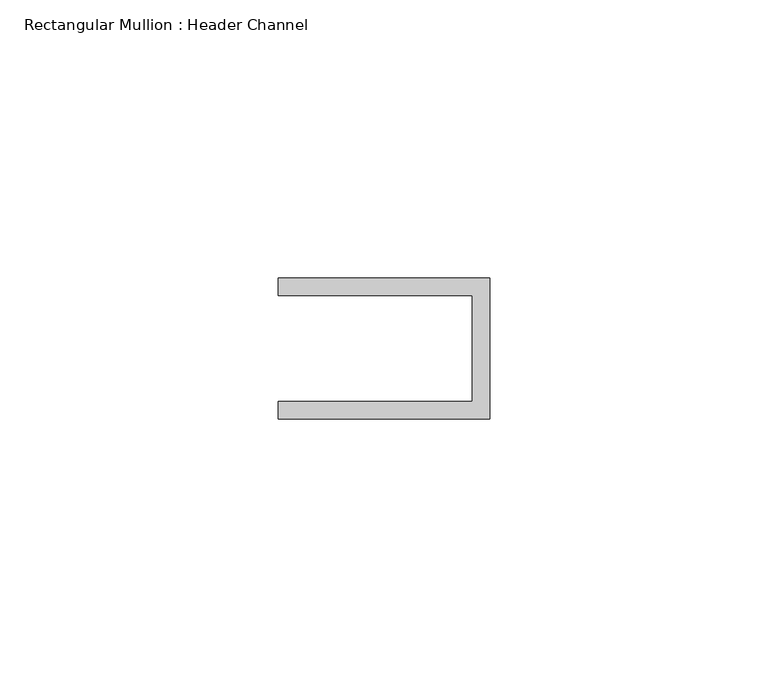
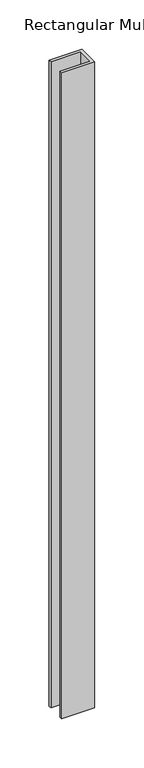
"""IFC4 building model written with IfcOpenShell, lengths in millimetres: member geometry, Rectangular Mullion : Header Channel."""

from ifc_helpers import new_model, si_unit, frame, origin, place, context, project, spatial, polyline, outline, extrude, source, transform, mapped, element, save


def rectangular_mullion_header_channel_80624e16(model_context):
    return source(origin(), model_context, "Body", "SweptSolid", [
        extrude(outline(polyline([(0.0, -12.7), (-38.1, -12.7), (-38.1, -9.525), (-3.175, -9.525), (-3.175, 9.525), (-38.1, 9.525), (-38.1, 12.7), (0.0, 12.7), (0.0, -12.7)])), frame((0.0, 0.0, -797.4590998), z_axis=(0.0, 0.0, 1.0), x_axis=(1.0, 0.0, 0.0)), (0.0, 0.0, 1.0), 797.4590998),
    ])


if __name__ == "__main__":
    model = new_model("IFC4")
    model_context = context("Model", 3, world=origin())
    ifc_project = project(units=[si_unit("LENGTHUNIT", "METRE", prefix="MILLI")], contexts=[model_context])
    site = spatial("IfcSite", under=ifc_project)
    building = spatial("IfcBuilding", under=site)
    placement = place(None, origin())
    rectangular_mullion_header_channel_shape = rectangular_mullion_header_channel_80624e16(model_context)
    element("IfcMember", 1, ObjectType="Rectangular Mullion : Header Channel", at=placement, inside=building, context=model_context, shape_type="MappedRepresentation", body=[
        mapped(rectangular_mullion_header_channel_shape, transform((0.0, 0.0, 0.0), x_axis=(1.0, 0.0, 0.0), y_axis=(0.0, 1.0, 0.0), z_axis=(0.0, 0.0, 1.0))),
    ])
    save(model, "model.ifc")

# Revit data of these elements
# Type "Rectangular Mullion : Header Channel"
#   built-in parameter 1007322 = 0.0833333 (stored number, unit not read)
#   built-in parameter 1007321 = -0.03125 (stored number, unit not read)
#   built-in parameter 1007320 = 0.0416667 (stored number, unit not read)
# Element 1 (IfcMember, "Rectangular Mullion : Header Channel")
#   Materials on its faces: "ALUM"
# Materials
#   "ALUM": class "Generic", colour RGB 157 157 157, transparency 0, Cost = 0
